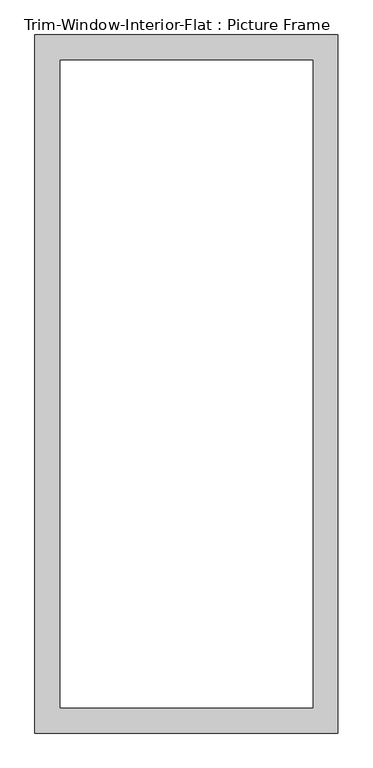
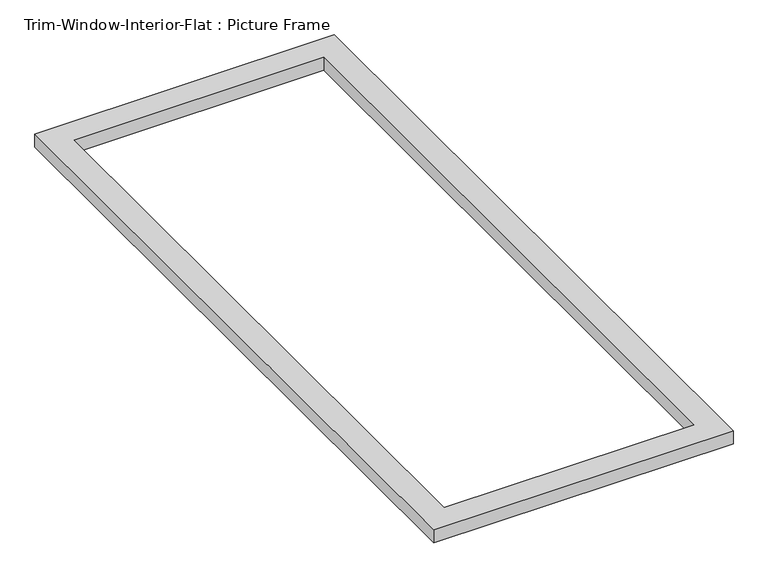
"""IFC4 building model written with IfcOpenShell, lengths in millimetres: proxy geometry, Trim-Window-Interior-Flat : Picture Frame."""

from ifc_helpers import new_model, si_unit, origin, origin_with_axes, place, context, project, spatial, polyline, outline, extrude, source, transform, mapped, element, save


def trim_window_interior_flat_picture_frame_5ec1ed24(model_context):
    return source(origin(), model_context, "Body", "SweptSolid", [
        extrude(outline(polyline([(344.45, 44.45), (344.45, -1544.45), (-344.45, -1544.45), (-344.45, 44.45), (344.45, 44.45)]), holes=[polyline([(287.3, -12.7), (-287.3, -12.7), (-287.3, -1487.3), (287.3, -1487.3), (287.3, -12.7)])]), origin_with_axes(), (0.0, 0.0, 1.0), 31.75),
    ])


if __name__ == "__main__":
    model = new_model("IFC4")
    model_context = context("Model", 3, world=origin())
    ifc_project = project(units=[si_unit("LENGTHUNIT", "METRE", prefix="MILLI")], contexts=[model_context])
    site = spatial("IfcSite", under=ifc_project)
    building = spatial("IfcBuilding", under=site)
    placement = place(None, origin())
    trim_window_interior_flat_picture_frame_shape = trim_window_interior_flat_picture_frame_5ec1ed24(model_context)
    element("IfcBuildingElementProxy", 1, Name="Trim-Window-Interior-Flat : Picture Frame", ObjectType="Trim-Window-Interior-Flat : Picture Frame", at=placement, inside=building, context=model_context, shape_type="MappedRepresentation", body=[
        mapped(trim_window_interior_flat_picture_frame_shape, transform((0.0, 0.0, 0.0), x_axis=(1.0, 0.0, 0.0), y_axis=(0.0, 1.0, 0.0), z_axis=(0.0, 0.0, 1.0))),
    ])
    save(model, "model.ifc")

# Revit data of these elements
# Type "Trim-Window-Interior-Flat : Picture Frame"
#   Trim Thickness_Picture Frame = 3.175 cm
#   Trim Width = 5.715 cm
#   Trim Thickness_with Sill = 1.905 cm
#   Sill Thickness = 3.175 cm
#   Opening Width [instance default] = 60.96 cm
#   Opening Height [instance default] = 91.44 cm
#   Default Elevation = 121.92 cm
#   Sill = no
#   Picture Frame = yes
#   Trim Material [instance default] = none
# Element 1 (IfcBuildingElementProxy, "Trim-Window-Interior-Flat : Picture Frame")
#   Opening Width = 60 cm
#   Opening Height = 150 cm
#   Trim Material = Wood - Stained
#   Materials on its faces: "Wood - Stained"
# Materials
#   "Wood - Stained": class "Wood", colour RGB 224 178 126, transparency 0, Cost = 0
